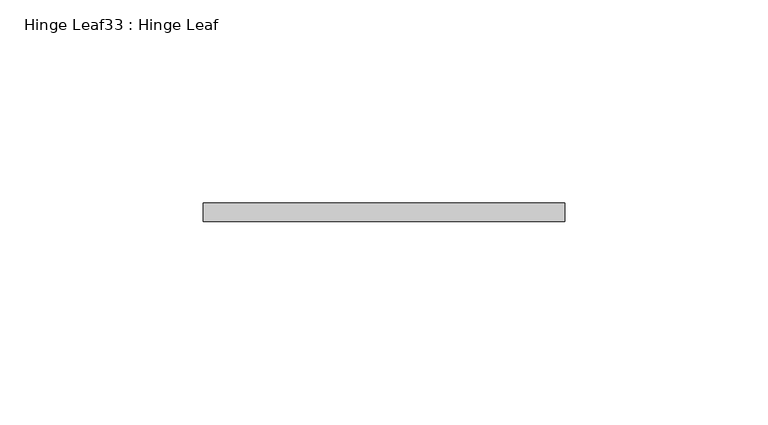
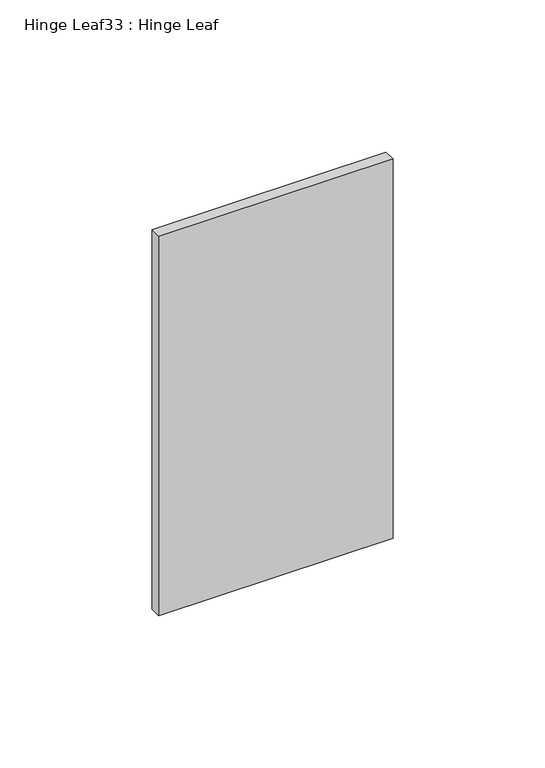
"""IFC4 building model written with IfcOpenShell, lengths in millimetres: proxy geometry, Hinge Leaf33 : Hinge Leaf."""

from ifc_helpers import new_model, si_unit, frame, origin, place, context, project, spatial, polyline, outline, extrude, source, transform, mapped, element, save


def hinge_leaf33_hinge_leaf_106c3047(model_context):
    return source(origin(), model_context, "Body", "SweptSolid", [
        extrude(outline(polyline([(587327.7934739, -533988.7163841), (587327.7934739, -533984.1443841), (587416.6934739, -533984.1443841), (587416.6934739, -533988.7163841), (587327.7934739, -533988.7163841)])), frame((0.0, 0.0, 311.15), z_axis=(0.0, 0.0, 1.0), x_axis=(1.0, 0.0, 0.0)), (0.0, 0.0, 1.0), 152.4),
    ])


if __name__ == "__main__":
    model = new_model("IFC4")
    model_context = context("Model", 3, world=origin())
    ifc_project = project(units=[si_unit("LENGTHUNIT", "METRE", prefix="MILLI")], contexts=[model_context])
    site = spatial("IfcSite", under=ifc_project)
    building = spatial("IfcBuilding", under=site)
    placement = place(None, origin())
    hinge_leaf33_hinge_leaf_shape = hinge_leaf33_hinge_leaf_106c3047(model_context)
    element("IfcBuildingElementProxy", 1, Name="Hinge Leaf33 : Hinge Leaf", ObjectType="Hinge Leaf33 : Hinge Leaf", at=placement, inside=building, context=model_context, shape_type="MappedRepresentation", body=[
        mapped(hinge_leaf33_hinge_leaf_shape, transform((0.0, 0.0, 0.0), x_axis=(1.0, 0.0, 0.0), y_axis=(0.0, 1.0, 0.0), z_axis=(0.0, 0.0, 1.0))),
    ])
    save(model, "model.ifc")

# Revit data of these elements
# Element 1 (IfcBuildingElementProxy, "Hinge Leaf33 : Hinge Leaf")
#   Materials on its faces: "6\"X6\" WELD-ON STL BUTT HINGE"
# Materials
#   "6\"X6\" WELD-ON STL BUTT HINGE": class "Metal", colour RGB 189 187 185, transparency 0, Description = "Carbon steel", Cost = 0
